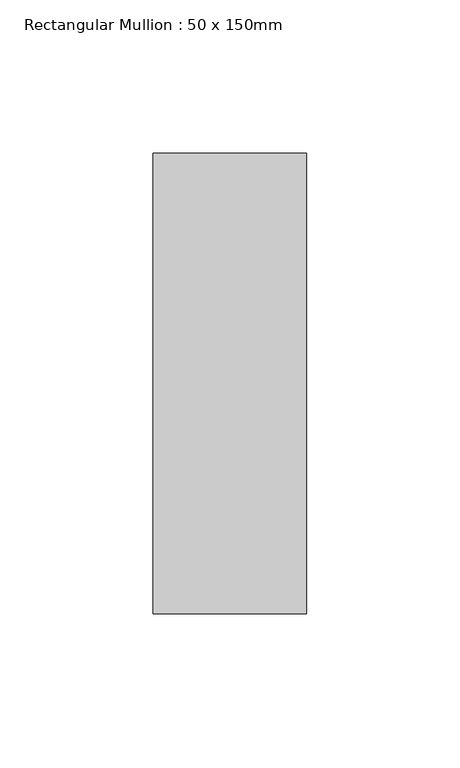
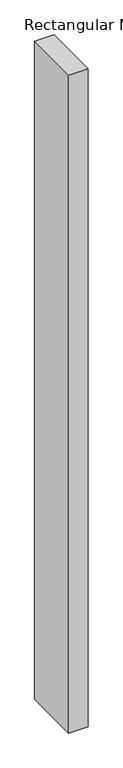
"""IFC4 building model written with IfcOpenShell, lengths in millimetres: member geometry, Rectangular Mullion : 50 x 150mm."""

import ifcopenshell
import ifcopenshell.guid

model = None  # the IFC model being written
_history = None  # IfcOwnerHistory: only IFC2X3 demands one
_inside = {}  # id of a spatial element -> (the spatial element, [elements in it])
_under = {}  # id of a project, library or spatial element -> (it, [spatial elements below it])
_declared = {}  # id of a project -> (the project, [libraries it declares])
_typed = {}  # id of a type object -> (the type object, [elements of that type])
_made_of = {}  # id of a material, layer set ... -> (it, [elements and type objects made of it])


def new_model(schema):
    """Start an empty IFC model of exactly this schema.

    Asked for "IFC4X3", IfcOpenShell would pick the latest addendum, in which some entities
    have other attributes; the version numbers below select the first issue.
    IFC2X3 requires an IfcOwnerHistory on every rooted entity: one is made here for all.
    """
    global model, _history
    if schema == "IFC4X3":
        model = ifcopenshell.file(schema_version=(4, 3, 0, 0))
    else:
        model = ifcopenshell.file(schema=schema)
    _inside.clear()
    _under.clear()
    _declared.clear()
    _typed.clear()
    _made_of.clear()
    _history = None
    if model.schema == "IFC2X3":
        org = make("IfcOrganization", Name="unknown")
        user = make(
            "IfcPersonAndOrganization",
            ThePerson=make("IfcPerson", FamilyName="unknown"),
            TheOrganization=org,
        )
        app = make(
            "IfcApplication",
            ApplicationDeveloper=org,
            Version="unknown",
            ApplicationFullName="unknown",
            ApplicationIdentifier="unknown",
        )
        _history = make(
            "IfcOwnerHistory",
            OwningUser=user,
            OwningApplication=app,
            ChangeAction="ADDED",
            CreationDate=0,
        )
    return model


def make(cls, **values):
    """One entity of the class cls with the attributes given. An attribute that is None is left unset."""
    return model.create_entity(
        cls, **{name: value for name, value in values.items() if value is not None}
    )


def rooted(cls, **values):
    """An entity with a GlobalId (a new one), such as an element, a storey or a relation."""
    return make(cls, GlobalId=ifcopenshell.guid.new(), OwnerHistory=_history, **values)


def si_unit(unit_type, name, prefix=None):
    """IfcSIUnit, for example si_unit("LENGTHUNIT", "METRE", prefix="MILLI")."""
    return make("IfcSIUnit", UnitType=unit_type, Prefix=prefix, Name=name)


def assignment(units):
    """IfcUnitAssignment: the units of a project."""
    return None if units is None else make("IfcUnitAssignment", Units=units)


def point(xyz):
    """IfcCartesianPoint."""
    return None if xyz is None else make("IfcCartesianPoint", Coordinates=xyz)


def direction(xyz):
    """IfcDirection."""
    return None if xyz is None else make("IfcDirection", DirectionRatios=xyz)


def frame(location, z_axis=None, x_axis=None):
    """IfcAxis2Placement3D, a coordinate frame: its origin and axes. An axis left out is left unset."""
    return make(
        "IfcAxis2Placement3D",
        Location=point(location),
        Axis=direction(z_axis),
        RefDirection=direction(x_axis),
    )


def origin():
    """The frame at (0, 0, 0) with its axes left unset."""
    return frame((0.0, 0.0, 0.0))


def place(relative_to, where):
    """IfcLocalPlacement: puts the frame where relative to a parent placement (None: the world)."""
    return make(
        "IfcLocalPlacement", PlacementRelTo=relative_to, RelativePlacement=where
    )


def context(
    kind, dimensions, precision=None, world=None, true_north=None, identifier=None
):
    """IfcGeometricRepresentationContext, for example the 3D "Model" context."""
    return make(
        "IfcGeometricRepresentationContext",
        ContextIdentifier=identifier,
        ContextType=kind,
        CoordinateSpaceDimension=dimensions,
        Precision=precision,
        WorldCoordinateSystem=world,
        TrueNorth=true_north,
    )


def project(units=None, contexts=None):
    """IfcProject with its units and contexts."""
    return rooted(
        "IfcProject",
        Name="project",
        RepresentationContexts=contexts,
        UnitsInContext=assignment(units),
    )


def spatial(cls, under=None, at=None, **own):
    """A site, building, storey or space (cls), placed at a placement, below another one or the project."""
    s = rooted(cls, ObjectPlacement=at, **own)
    if under is not None:
        _under.setdefault(under.id(), (under, []))[1].append(s)
    return s


def polyline(points):
    """IfcPolyline through the points."""
    return make("IfcPolyline", Points=[point(p) for p in points])


def outline(outer, holes=None, kind="AREA"):
    """IfcArbitraryClosedProfileDef: a profile drawn as a closed curve; with holes, ...WithVoids."""
    if holes is None:
        return make("IfcArbitraryClosedProfileDef", ProfileType=kind, OuterCurve=outer)
    return make(
        "IfcArbitraryProfileDefWithVoids",
        ProfileType=kind,
        OuterCurve=outer,
        InnerCurves=holes,
    )


def extrude(swept, where, along, depth):
    """IfcExtrudedAreaSolid: the profile swept, set in the frame where, extruded along a direction by depth."""
    return make(
        "IfcExtrudedAreaSolid",
        SweptArea=swept,
        Position=where,
        ExtrudedDirection=direction(along),
        Depth=depth,
    )


def shape(context_of_items, identifier, shape_type, items):
    """IfcShapeRepresentation: the items that make up one representation, for example the "Body"."""
    return make(
        "IfcShapeRepresentation",
        ContextOfItems=context_of_items,
        RepresentationIdentifier=identifier,
        RepresentationType=shape_type,
        Items=items,
    )


def source(mapping_origin, context_of_items, identifier, shape_type, items):
    """IfcRepresentationMap: a shape defined once, which mapped items show again and again."""
    return make(
        "IfcRepresentationMap",
        MappingOrigin=mapping_origin,
        MappedRepresentation=shape(context_of_items, identifier, shape_type, items),
    )


def transform(
    local_origin,
    x_axis=None,
    y_axis=None,
    z_axis=None,
    scale=None,
    scale2=None,
    scale3=None,
    uniform=True,
):
    """IfcCartesianTransformationOperator3D, or its non-uniform kind. x_axis, y_axis, z_axis: its Axis1, 2, 3."""
    if uniform:
        return make(
            "IfcCartesianTransformationOperator3D",
            Axis1=direction(x_axis),
            Axis2=direction(y_axis),
            LocalOrigin=point(local_origin),
            Scale=scale,
            Axis3=direction(z_axis),
        )
    return make(
        "IfcCartesianTransformationOperator3DnonUniform",
        Axis1=direction(x_axis),
        Axis2=direction(y_axis),
        LocalOrigin=point(local_origin),
        Scale=scale,
        Axis3=direction(z_axis),
        Scale2=scale2,
        Scale3=scale3,
    )


def mapped(mapping_source, mapping_target):
    """IfcMappedItem: shows the shape of a source again, moved by a transform."""
    return make(
        "IfcMappedItem", MappingSource=mapping_source, MappingTarget=mapping_target
    )


def made_of(thing, what):
    """Note that an element or type object is made of a material, layer set ...; save() writes the relation."""
    if what is not None:
        _made_of.setdefault(what.id(), (what, []))[1].append(thing)
    return thing


def element(
    cls,
    number,
    at=None,
    inside=None,
    cuts=None,
    type_object=None,
    material=None,
    context=None,
    identifier="Body",
    shape_type=None,
    held_by="IfcProductDefinitionShape",
    body=None,
    shapes=None,
    **own,
):
    """One element of the class cls, such as IfcWall. Its Tag is "e" and its number.

    at: its placement. inside: the storey or other place that contains it. cuts: it is an
    opening in that element (IfcRelVoidsElement). A single representation is given by context,
    identifier, shape_type and body (its items); several are given by shapes. held_by: the class
    of the entity that holds the representations. save() writes the other relations.
    """
    e = rooted(cls, Tag="e%d" % number, ObjectPlacement=at, **own)
    if body is not None:
        shapes = [shape(context, identifier, shape_type, body)]
    if shapes is not None:
        e.Representation = make(held_by, Representations=shapes)
    if inside is not None:
        _inside.setdefault(inside.id(), (inside, []))[1].append(e)
    if cuts is not None:
        rooted(
            "IfcRelVoidsElement", RelatingBuildingElement=cuts, RelatedOpeningElement=e
        )
    if type_object is not None:
        _typed.setdefault(type_object.id(), (type_object, []))[1].append(e)
    return made_of(e, material)


def aggregate(whole, parts):
    """IfcRelAggregates: a whole, such as a stair, and the parts it consists of."""
    return rooted("IfcRelAggregates", RelatingObject=whole, RelatedObjects=parts)


def save(model, path):
    """Write the relations noted so far, then the file.

    IfcRelAggregates (storeys below a building ...), IfcRelContainedInSpatialStructure (elements
    in a storey), IfcRelDefinesByType, IfcRelAssociatesMaterial and IfcRelDeclares: one each for
    every whole, place, type object, material and project.
    """
    for whole, parts in _under.values():
        aggregate(whole, parts)
    for where, things in _inside.values():
        rooted(
            "IfcRelContainedInSpatialStructure",
            RelatedElements=things,
            RelatingStructure=where,
        )
    for kind, things in _typed.values():
        rooted("IfcRelDefinesByType", RelatedObjects=things, RelatingType=kind)
    for what, things in _made_of.values():
        rooted("IfcRelAssociatesMaterial", RelatedObjects=things, RelatingMaterial=what)
    for by, libraries in _declared.values():
        rooted("IfcRelDeclares", RelatingContext=by, RelatedDefinitions=libraries)
    model.write(path)


def rectangular_mullion_50_x_150mm_1e81bce4(model_context):
    return source(origin(), model_context, "Body", "SweptSolid", [
        extrude(outline(polyline([(0.0, 75.0), (0.0, -75.0), (-50.0, -75.0), (-50.0, 75.0), (0.0, 75.0)])), frame((0.0, 0.0, -1775.8970067), z_axis=(0.0, 0.0, 1.0), x_axis=(1.0, 0.0, 0.0)), (0.0, 0.0, 1.0), 1775.8970067),
    ])


if __name__ == "__main__":
    model = new_model("IFC4")
    model_context = context("Model", 3, world=origin())
    ifc_project = project(units=[si_unit("LENGTHUNIT", "METRE", prefix="MILLI")], contexts=[model_context])
    site = spatial("IfcSite", under=ifc_project)
    building = spatial("IfcBuilding", under=site)
    placement = place(None, origin())
    rectangular_mullion_50_x_150mm_shape = rectangular_mullion_50_x_150mm_1e81bce4(model_context)
    element("IfcMember", 1, ObjectType="Rectangular Mullion : 50 x 150mm", at=placement, inside=building, context=model_context, shape_type="MappedRepresentation", body=[
        mapped(rectangular_mullion_50_x_150mm_shape, transform((0.0, 0.0, 0.0), x_axis=(1.0, 0.0, 0.0), y_axis=(0.0, 1.0, 0.0), z_axis=(0.0, 0.0, 1.0))),
    ])
    save(model, "model.ifc")

# Revit data of these elements
# Type "Rectangular Mullion : 50 x 150mm"
#   Keynote = "H11"
#   built-in parameter 1007304 = 0.492126 (stored number, unit not read)
#   built-in parameter 1007301 = 0.082021 (stored number, unit not read)
#   built-in parameter 1007300 = 0.082021 (stored number, unit not read)
# Element 1 (IfcMember, "Rectangular Mullion : 50 x 150mm")
#   Materials on its faces: "Aluminium"
# Materials
#   "Aluminium": class "Metal", colour RGB 247 247 247, transparency 0, Description = "Aluminium 6061", Cost = 0
